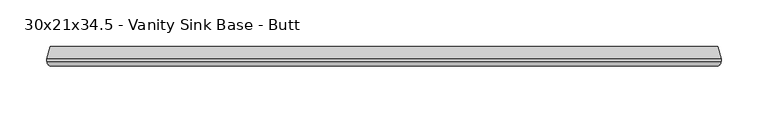
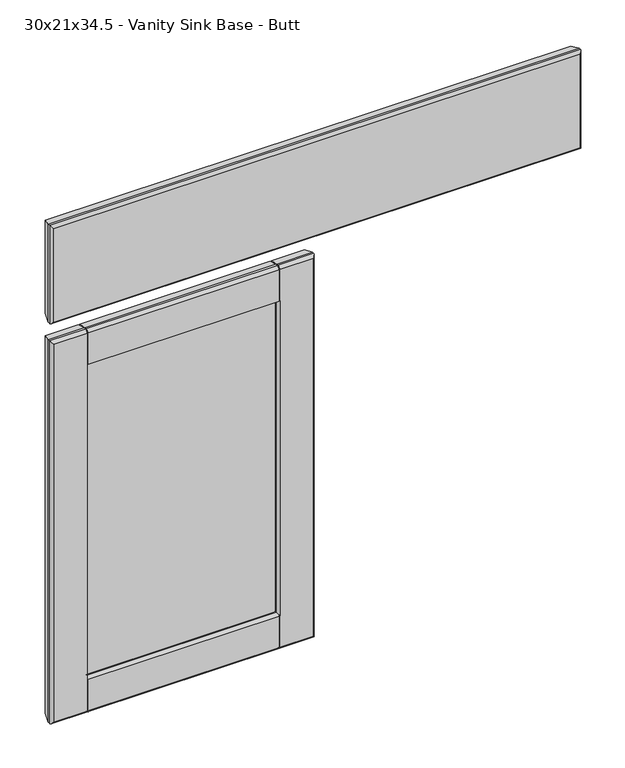
"""IFC4 building model written with IfcOpenShell, lengths in millimetres: furniture geometry, Cabinet-Base-Merillat-Double_Door-Marlin : 30x21x34.5 - Vanity Sink Base - Butt."""

from ifc_helpers import new_model, si_unit, frame, origin, place, context, project, spatial, polyline, circle_curve, ellipse_curve, outline, extrude, source, transform, mapped, element, save
from ifc_brep_helpers import plane_surface, cylinder_surface, advanced_brep


def furniture_30x21x34_5_vanity_sink_base_butt_accc5f2d(model_context):
    return source(origin(), model_context, "Body", "SolidModel", [
        advanced_brep(
        [(-336.9408026, -629.92, 847.8035075), (-336.9408026, -629.92, 714.2964925), (374.4162124, -629.92, 714.2964925), (374.4162124, -629.92, 847.8035075), (-336.5320951, -609.6, 714.7052), (-336.5320951, -609.6, 847.3948), (374.0075049, -609.6, 847.3948), (374.0075049, -609.6, 714.7052), (-340.0372951, -625.4496, 850.9), (-340.0372951, -622.681, 850.9), (-340.0372951, -622.681, 711.2), (-340.0372951, -625.4496, 711.2), (377.5127049, -622.681, 711.2), (377.5127049, -625.4496, 711.2), (377.5127049, -622.681, 850.9), (377.5127049, -625.4496, 850.9)],
        [
            (0, 1),
            (1, 2),
            (2, 3),
            (3, 0),
            (4, 5),
            (5, 6),
            (6, 7),
            (7, 4),
            (8, 9),
            (9, 10),
            (10, 11),
            (11, 8),
            (10, 12),
            (12, 13),
            (13, 11),
            (12, 14),
            (14, 15),
            (15, 13),
            (8, 15),
            (14, 9),
            (11, 1, ellipse_curve(frame((-335.2620951, -625.4496, 715.9752), z_axis=(-0.7071067811865475, 0.0, 0.7071067811865475), x_axis=(-0.7071067811865474, 0.0, -0.7071067811865476)), 6.7531526, 4.7752)),
            (0, 8, ellipse_curve(frame((-335.2620951, -625.4496, 846.1248), z_axis=(-0.7071067811865475, 0.0, -0.7071067811865475), x_axis=(0.7071067811865474, 0.0, -0.7071067811865476)), 6.7531526, 4.7752)),
            (4, 10),
            (9, 5),
            (13, 2, ellipse_curve(frame((372.7375049, -625.4496, 715.9752), z_axis=(-0.7071067811865475, 0.0, -0.7071067811865475), x_axis=(0.7071067811865476, 0.0, -0.7071067811865474)), 6.7531526, 4.7752)),
            (7, 12),
            (15, 3, ellipse_curve(frame((372.7375049, -625.4496, 846.1248), z_axis=(0.7071067811865475, 0.0, -0.7071067811865475), x_axis=(0.7071067811865474, 0.0, 0.7071067811865476)), 6.7531526, 4.7752)),
            (6, 14),
        ],
        [
            plane_surface(frame((-340.0372951, -629.92, 850.9), z_axis=(0.0, -1.0, 0.0), x_axis=(0.0, 0.0, -1.0))),
            plane_surface(frame((-340.0372951, -609.6, 850.9), z_axis=(0.0, 1.0, 0.0), x_axis=(0.0, 0.0, 1.0))),
            plane_surface(frame((-340.0372951, -629.92, 850.9), z_axis=(-1.0, 0.0, 0.0), x_axis=(0.0, 1.0, 0.0))),
            plane_surface(frame((-340.0372951, -629.92, 711.2), z_axis=(0.0, 0.0, -1.0), x_axis=(0.0, 1.0, 0.0))),
            plane_surface(frame((377.5127049, -629.92, 711.2), z_axis=(1.0, 0.0, 0.0), x_axis=(0.0, 1.0, 0.0))),
            plane_surface(frame((377.5127049, -629.92, 850.9), z_axis=(0.0, 0.0, 1.0), x_axis=(0.0, 1.0, 0.0))),
            cylinder_surface(frame((-335.2620951, -625.4496, 850.9), z_axis=(0.0, 0.0, -1.0), x_axis=(0.0, 1.0, 0.0)), 4.7752),
            plane_surface(frame((-340.0372951, -622.681, 850.9), z_axis=(-0.9659229350723619, 0.25882983502910506, 0.0), x_axis=(0.0, 0.0, -1.0))),
            cylinder_surface(frame((-340.0372951, -625.4496, 715.9752), z_axis=(1.0, 0.0, 0.0), x_axis=(0.0, 1.0, 0.0)), 4.7752),
            plane_surface(frame((-340.0372951, -622.681, 711.2), z_axis=(0.0, 0.25882983502910506, -0.9659229350723619), x_axis=(1.0, 0.0, 0.0))),
            cylinder_surface(frame((372.7375049, -625.4496, 711.2), z_axis=(0.0, 0.0, 1.0), x_axis=(0.0, 1.0, 0.0)), 4.7752),
            plane_surface(frame((377.5127049, -622.681, 711.2), z_axis=(0.9659229350723619, 0.25882983502910506, 0.0), x_axis=(0.0, 0.0, 1.0))),
            cylinder_surface(frame((377.5127049, -625.4496, 846.1248), z_axis=(-1.0, 0.0, 0.0), x_axis=(0.0, 1.0, 0.0)), 4.7752),
            plane_surface(frame((377.5127049, -622.681, 850.9), z_axis=(0.0, 0.25882983502910506, 0.9659229350723619), x_axis=(-1.0, 0.0, 0.0))),
        ],
        [
            (0, [[1, 2, 3, 4]]),
            (1, [[5, 6, 7, 8]]),
            (2, [[9, 10, 11, 12]]),
            (3, [[-11, 13, 14, 15]]),
            (4, [[-14, 16, 17, 18]]),
            (5, [[-9, 19, -17, 20]]),
            (6, [[21, -1, 22, -12]]),
            (7, [[23, -10, 24, -5]]),
            (8, [[-21, -15, 25, -2]]),
            (9, [[-23, -8, 26, -13]]),
            (10, [[-25, -18, 27, -3]]),
            (11, [[-26, -7, 28, -16]]),
            (12, [[-22, -4, -27, -19]]),
            (13, [[-24, -20, -28, -6]]),
        ],
    ),
        advanced_brep(
        [(-340.0372951, -625.4496, 685.8), (-340.0372951, -625.4496, 139.7), (-336.9408026, -629.92, 142.7964925), (-336.9408026, -629.92, 682.7035075), (-340.0372951, -622.681, 685.8), (-340.0372951, -622.681, 139.7), (-336.5320951, -609.6, 682.2948), (-336.5320951, -609.6, 143.2052), (-291.8361323, -609.6, 637.5988372), (-291.4660006, -610.39375, 637.2287055), (-289.3848416, -614.85681, 635.1475465), (-289.3848416, -614.85681, 190.3524535), (-291.4660006, -610.39375, 188.2712945), (-291.8361323, -609.6, 187.9011628), (-290.784611, -617.0969093, 636.547316), (-290.784611, -617.0969093, 188.952684), (-305.1122951, -617.347, 650.875), (-305.1122951, -617.347, 174.625), (-305.1122951, -622.173, 650.875), (-305.1122951, -622.173, 174.625), (-290.784611, -622.4230907, 636.547316), (-290.784611, -622.4230907, 188.952684), (-289.3848416, -624.66319, 635.1475465), (-289.3848416, -624.66319, 190.3524535), (-291.4660006, -629.12625, 637.2287055), (-291.8332649, -629.9138508, 637.5959698), (-291.8361323, -629.92, 187.9011628), (-291.4660006, -629.12625, 188.2712945), (14.0537124, -629.92, 142.7964925), (-31.0140137, -629.92, 142.7964925), (-31.0140137, -625.4496, 139.7), (17.1502049, -625.4496, 139.7), (-291.8332649, -625.4496, 139.7), (-291.8332649, -629.92, 142.7964925), (-290.2457649, -625.4496, 139.7), (-32.6015137, -625.4496, 139.7), (-32.6015137, -629.92, 142.7964925), (-290.2457649, -629.92, 142.7964925), (-31.0140137, -622.681, 139.7), (17.1502049, -622.681, 139.7), (-291.8332649, -622.681, 139.7), (-290.2457649, -622.681, 139.7), (-32.6015137, -622.681, 139.7), (-31.0140137, -609.6, 143.2052), (13.6450049, -609.6, 143.2052), (-290.2457649, -609.6, 143.2052), (-32.6015137, -609.6, 143.2052), (-291.8332649, -609.6, 143.2052), (-33.5022486, -614.85681, 190.3524535), (-31.4210895, -610.39375, 188.2712945), (-32.6015137, -610.39375, 188.2712945), (-32.6015137, -609.6, 187.9011628), (-290.2457649, -609.6, 187.9011628), (-290.2457649, -610.39375, 188.2712945), (-32.1024791, -617.0969093, 188.952684), (-17.7747951, -617.347, 174.625), (-17.7747951, -622.173, 174.625), (-32.1024791, -622.4230907, 188.952684), (-33.5022486, -624.66319, 190.3524535), (-290.2457649, -629.12625, 188.2712945), (-290.2457649, -629.92, 187.9011628), (-32.6015137, -629.92, 187.9011628), (-32.6015137, -629.12625, 188.2712945), (-31.4210895, -629.12625, 188.2712945), (17.1502049, -625.4496, 685.8), (14.0537124, -629.92, 682.7035075), (17.1502049, -622.681, 685.8), (13.6450049, -609.6, 682.2948), (-31.0509578, -609.6, 187.9011628), (-33.5022486, -614.85681, 635.1475465), (-31.4210895, -610.39375, 637.2287055), (-31.0509578, -609.6, 637.5988372), (-32.1024791, -617.0969093, 636.547316), (-17.7747951, -617.347, 650.875), (-17.7747951, -622.173, 650.875), (-32.1024791, -622.4230907, 636.547316), (-33.5022486, -624.66319, 635.1475465), (-31.0509578, -629.92, 187.9011628), (-31.0509578, -629.92, 637.5988372), (-31.4210895, -629.12625, 637.2287055), (-291.8332649, -629.92, 682.7035075), (-291.8332649, -625.4496, 685.8), (-31.0140137, -625.4496, 685.8), (-31.0140137, -629.92, 682.7035075), (-32.6015137, -625.4496, 685.8), (-290.2457649, -625.4496, 685.8), (-290.2457649, -629.92, 682.7035075), (-32.6015137, -629.92, 682.7035075), (-291.8332649, -622.681, 685.8), (-31.0140137, -622.681, 685.8), (-32.6015137, -622.681, 685.8), (-290.2457649, -622.681, 685.8), (-291.8332649, -609.6, 682.2948), (-31.0140137, -609.6, 682.2948), (-32.6015137, -609.6, 682.2948), (-290.2457649, -609.6, 682.2948), (-32.6015137, -609.6, 637.5988372), (-290.2457649, -609.6, 637.5988372), (-290.2457649, -610.39375, 637.2287055), (-32.6015137, -610.39375, 637.2287055), (-32.6015137, -629.12625, 637.2287055), (-32.6015137, -629.92, 637.5988372), (-290.2457649, -629.92, 637.5988372), (-290.2457649, -629.12625, 637.2287055), (-32.6015137, -629.12625, 682.5526052), (-32.6015137, -625.4496, 685.00625), (-32.6015137, -622.7855037, 685.00625), (-32.6015137, -610.39375, 681.6857412), (-31.0140137, -610.39375, 637.2287055), (-31.0140137, -610.39375, 681.6857412), (-31.0140137, -622.7855037, 685.00625), (-31.0140137, -625.4496, 685.00625), (-31.0140137, -629.12625, 682.5526052), (-31.0140137, -629.12625, 637.2287055), (-291.8332649, -629.12625, 637.2287055), (-291.8332649, -629.12625, 682.5526052), (-291.8332649, -625.4496, 685.00625), (-291.8332649, -622.7855037, 685.00625), (-291.8332649, -610.39375, 681.6857412), (-291.8332649, -610.39375, 637.2287055), (-290.2457649, -610.39375, 681.6857412), (-290.2457649, -622.7855037, 685.00625), (-290.2457649, -625.4496, 685.00625), (-290.2457649, -629.12625, 682.5526052), (-291.8332649, -610.39375, 188.2712945), (-291.8332649, -610.39375, 143.8142588), (-291.8332649, -622.7855037, 140.49375), (-291.8332649, -625.4496, 140.49375), (-291.8332649, -629.12625, 142.9473948), (-291.8332649, -629.12625, 188.2712945), (-290.2457649, -629.12625, 142.9473948), (-290.2457649, -625.4496, 140.49375), (-290.2457649, -622.7855037, 140.49375), (-290.2457649, -610.39375, 143.8142588), (-32.6015137, -610.39375, 143.8142588), (-32.6015137, -622.7855037, 140.49375), (-32.6015137, -625.4496, 140.49375), (-32.6015137, -629.12625, 142.9473948), (-31.0140137, -629.12625, 188.2712945), (-31.0140137, -629.12625, 142.9473948), (-31.0140137, -625.4496, 140.49375), (-31.0140137, -622.7855037, 140.49375), (-31.0140137, -610.39375, 143.8142588), (-31.0140137, -610.39375, 188.2712945)],
        [
            (0, 1),
            (1, 2, ellipse_curve(frame((-335.2620951, -625.4496, 144.4752), z_axis=(-0.7071067811865475, 0.0, 0.7071067811865475), x_axis=(0.7071067811865474, 0.0, 0.7071067811865476)), 6.7531526, 4.7752)),
            (2, 3),
            (3, 0, ellipse_curve(frame((-335.2620951, -625.4496, 681.0248), z_axis=(-0.7071067811865475, 0.0, -0.7071067811865475), x_axis=(-0.7071067811865474, 0.0, 0.7071067811865476)), 6.7531526, 4.7752)),
            (0, 4),
            (4, 5),
            (5, 1),
            (4, 6),
            (6, 7),
            (7, 5),
            (8, 9),
            (9, 10),
            (10, 11),
            (11, 12),
            (12, 13),
            (13, 8),
            (10, 14, ellipse_curve(frame((-290.8120951, -615.5223492, 636.5748), z_axis=(-0.7071067811865475, 0.0, -0.7071067811865475), x_axis=(-0.7071067811865474, 0.0, 0.7071067811865476)), 2.2271035, 1.5748)),
            (14, 15),
            (15, 11, ellipse_curve(frame((-290.8120951, -615.5223492, 188.9252), z_axis=(-0.7071067811865475, 0.0, 0.7071067811865475), x_axis=(0.7071067811865474, 0.0, 0.7071067811865476)), 2.2271035, 1.5748)),
            (14, 16),
            (16, 17),
            (17, 15),
            (16, 18),
            (18, 19),
            (19, 17),
            (18, 20),
            (20, 21),
            (21, 19),
            (20, 22, ellipse_curve(frame((-290.8120951, -623.9976508, 636.5748), z_axis=(-0.7071067811865475, 0.0, -0.7071067811865475), x_axis=(-0.7071067811865474, 0.0, 0.7071067811865476)), 2.2271035, 1.5748)),
            (22, 23),
            (23, 21, ellipse_curve(frame((-290.8120951, -623.9976508, 188.9252), z_axis=(-0.7071067811865475, 0.0, 0.7071067811865475), x_axis=(0.7071067811865474, 0.0, 0.7071067811865476)), 2.2271035, 1.5748)),
            (22, 24),
            (24, 25),
            (25, 26),
            (26, 27),
            (27, 23),
            (28, 29),
            (29, 30, circle_curve(frame((-31.0140137, -625.4496, 144.4752), z_axis=(1.0, 0.0, 0.0), x_axis=(0.0, 1.0, 0.0)), 4.7752)),
            (30, 31),
            (31, 28, ellipse_curve(frame((12.3750049, -625.4496, 144.4752), z_axis=(-0.7071067811865475, 0.0, -0.7071067811865475), x_axis=(-0.7071067811865476, 0.0, 0.7071067811865474)), 6.7531526, 4.7752)),
            (1, 32),
            (32, 33, circle_curve(frame((-291.8332649, -625.4496, 144.4752), z_axis=(-1.0, 0.0, 0.0), x_axis=(0.0, 1.0, 0.0)), 4.7752)),
            (33, 2),
            (34, 35),
            (35, 36, circle_curve(frame((-32.6015137, -625.4496, 144.4752), z_axis=(-1.0, 0.0, 0.0), x_axis=(0.0, 1.0, 0.0)), 4.7752)),
            (36, 37),
            (37, 34, circle_curve(frame((-290.2457649, -625.4496, 144.4752), z_axis=(1.0, 0.0, 0.0), x_axis=(0.0, 1.0, 0.0)), 4.7752)),
            (30, 38),
            (38, 39),
            (39, 31),
            (5, 40),
            (40, 32),
            (41, 42),
            (42, 35),
            (34, 41),
            (38, 43),
            (43, 44),
            (44, 39),
            (45, 46),
            (46, 42),
            (41, 45),
            (7, 47),
            (47, 40),
            (48, 49),
            (49, 50),
            (50, 51),
            (51, 52),
            (52, 53),
            (53, 12),
            (11, 48),
            (15, 54),
            (54, 48, ellipse_curve(frame((-32.0749951, -615.5223492, 188.9252), z_axis=(-0.7071067811865475, 0.0, -0.7071067811865475), x_axis=(-0.7071067811865476, 0.0, 0.7071067811865474)), 2.2271035, 1.5748)),
            (17, 55),
            (55, 54),
            (19, 56),
            (56, 55),
            (21, 57),
            (57, 56),
            (23, 58),
            (58, 57, ellipse_curve(frame((-32.0749951, -623.9976508, 188.9252), z_axis=(-0.7071067811865475, 0.0, -0.7071067811865475), x_axis=(-0.7071067811865476, 0.0, 0.7071067811865474)), 2.2271035, 1.5748)),
            (27, 59),
            (59, 60),
            (60, 61),
            (61, 62),
            (62, 63),
            (63, 58),
            (31, 64),
            (64, 65, ellipse_curve(frame((12.3750049, -625.4496, 681.0248), z_axis=(0.7071067811865475, 0.0, -0.7071067811865475), x_axis=(-0.7071067811865474, 0.0, -0.7071067811865476)), 6.7531526, 4.7752)),
            (65, 28),
            (39, 66),
            (66, 64),
            (44, 67),
            (67, 66),
            (68, 49),
            (48, 69),
            (69, 70),
            (70, 71),
            (71, 68),
            (54, 72),
            (72, 69, ellipse_curve(frame((-32.0749951, -615.5223492, 636.5748), z_axis=(0.7071067811865475, 0.0, -0.7071067811865475), x_axis=(-0.7071067811865474, 0.0, -0.7071067811865476)), 2.2271035, 1.5748)),
            (55, 73),
            (73, 72),
            (56, 74),
            (74, 73),
            (57, 75),
            (75, 74),
            (58, 76),
            (76, 75, ellipse_curve(frame((-32.0749951, -623.9976508, 636.5748), z_axis=(0.7071067811865475, 0.0, -0.7071067811865475), x_axis=(-0.7071067811865474, 0.0, -0.7071067811865476)), 2.2271035, 1.5748)),
            (63, 77),
            (77, 78),
            (78, 79),
            (79, 76),
            (3, 80),
            (80, 81, circle_curve(frame((-291.8332649, -625.4496, 681.0248), z_axis=(-1.0, 0.0, 0.0), x_axis=(0.0, 1.0, 0.0)), 4.7752)),
            (81, 0),
            (64, 82),
            (82, 83, circle_curve(frame((-31.0140137, -625.4496, 681.0248), z_axis=(1.0, 0.0, 0.0), x_axis=(0.0, 1.0, 0.0)), 4.7752)),
            (83, 65),
            (84, 85),
            (85, 86, circle_curve(frame((-290.2457649, -625.4496, 681.0248), z_axis=(1.0, 0.0, 0.0), x_axis=(0.0, 1.0, 0.0)), 4.7752)),
            (86, 87),
            (87, 84, circle_curve(frame((-32.6015137, -625.4496, 681.0248), z_axis=(-1.0, 0.0, 0.0), x_axis=(0.0, 1.0, 0.0)), 4.7752)),
            (81, 88),
            (88, 4),
            (66, 89),
            (89, 82),
            (90, 91),
            (91, 85),
            (84, 90),
            (88, 92),
            (92, 6),
            (67, 93),
            (93, 89),
            (94, 95),
            (95, 91),
            (90, 94),
            (51, 46),
            (45, 52),
            (43, 68),
            (71, 93),
            (92, 8),
            (13, 47),
            (96, 97),
            (97, 95),
            (94, 96),
            (9, 98),
            (98, 97),
            (96, 99),
            (99, 70),
            (69, 10),
            (72, 14),
            (73, 16),
            (74, 18),
            (75, 20),
            (76, 22),
            (79, 100),
            (100, 101),
            (101, 102),
            (102, 103),
            (103, 24),
            (33, 26),
            (25, 80),
            (36, 61),
            (60, 37),
            (83, 78),
            (77, 29),
            (86, 102),
            (101, 87),
            (100, 104),
            (104, 105, circle_curve(frame((-32.6015137, -625.4496, 681.0248), z_axis=(-1.0, 0.0, 0.0), x_axis=(0.0, 0.0, 1.0)), 3.98145)),
            (105, 106),
            (106, 107),
            (107, 99),
            (71, 108),
            (108, 109),
            (109, 110),
            (110, 111),
            (111, 112, circle_curve(frame((-31.0140137, -625.4496, 681.0248), z_axis=(1.0, 0.0, 0.0), x_axis=(0.0, 0.0, 1.0)), 3.98145)),
            (112, 113),
            (113, 78),
            (113, 79),
            (112, 104),
            (111, 105),
            (110, 106),
            (109, 107),
            (108, 70),
            (25, 114),
            (114, 115),
            (115, 116, circle_curve(frame((-291.8332649, -625.4496, 681.0248), z_axis=(-1.0, 0.0, 0.0), x_axis=(0.0, 0.0, 1.0)), 3.98145)),
            (116, 117),
            (117, 118),
            (118, 119),
            (119, 8),
            (98, 120),
            (120, 121),
            (121, 122),
            (122, 123, circle_curve(frame((-290.2457649, -625.4496, 681.0248), z_axis=(1.0, 0.0, 0.0), x_axis=(0.0, 0.0, 1.0)), 3.98145)),
            (123, 103),
            (24, 114),
            (123, 115),
            (122, 116),
            (121, 117),
            (120, 118),
            (9, 119),
            (13, 124),
            (124, 125),
            (125, 126),
            (126, 127),
            (127, 128, circle_curve(frame((-291.8332649, -625.4496, 144.4752), z_axis=(-1.0, 0.0, 0.0), x_axis=(0.0, 0.0, 1.0)), 3.98145)),
            (128, 129),
            (129, 26),
            (59, 130),
            (130, 131, circle_curve(frame((-290.2457649, -625.4496, 144.4752), z_axis=(1.0, 0.0, 0.0), x_axis=(0.0, 0.0, 1.0)), 3.98145)),
            (131, 132),
            (132, 133),
            (133, 53),
            (12, 124),
            (133, 125),
            (132, 126),
            (131, 127),
            (130, 128),
            (27, 129),
            (50, 134),
            (134, 135),
            (135, 136),
            (136, 137, circle_curve(frame((-32.6015137, -625.4496, 144.4752), z_axis=(-1.0, 0.0, 0.0), x_axis=(0.0, 0.0, 1.0)), 3.98145)),
            (137, 62),
            (138, 139),
            (139, 140, circle_curve(frame((-31.0140137, -625.4496, 144.4752), z_axis=(1.0, 0.0, 0.0), x_axis=(0.0, 0.0, 1.0)), 3.98145)),
            (140, 141),
            (141, 142),
            (142, 143),
            (143, 68),
            (77, 138),
            (63, 138),
            (143, 49),
            (142, 134),
            (141, 135),
            (140, 136),
            (139, 137),
        ],
        [
            cylinder_surface(frame((-335.2620951, -625.4496, 685.8), z_axis=(0.0, 0.0, 1.0), x_axis=(0.0, 1.0, 0.0)), 4.7752),
            plane_surface(frame((-340.0372951, -625.4496, 685.8), z_axis=(-1.0, 0.0, 0.0), x_axis=(0.0, 0.0, -1.0))),
            plane_surface(frame((-340.0372951, -622.681, 685.8), z_axis=(-0.9659229350723619, 0.25882983502910506, 0.0), x_axis=(0.0, 0.0, -1.0))),
            plane_surface(frame((-291.8361323, -609.6, 637.5988372), z_axis=(0.9063077870366099, 0.4226182617407856, 0.0), x_axis=(0.0, 0.0, -1.0))),
            cylinder_surface(frame((-290.8120951, -615.5223492, 685.8), z_axis=(0.0, 0.0, 1.0000000000000002), x_axis=(0.01745240643729364, -0.9998476951563912, 0.0)), 1.5748),
            plane_surface(frame((-290.784611, -617.0969093, 636.547316), z_axis=(0.017452406437322144, -0.9998476951563906, 0.0), x_axis=(0.0, 0.0, -1.0))),
            plane_surface(frame((-305.1122951, -617.347, 650.875), z_axis=(1.0, 0.0, 0.0), x_axis=(0.0, 0.0, -1.0))),
            plane_surface(frame((-305.1122951, -622.173, 650.875), z_axis=(0.01745240643727848, 0.9998476951563914, 0.0), x_axis=(0.0, 0.0, -1.0))),
            cylinder_surface(frame((-290.8120951, -623.9976508, 685.8), z_axis=(0.0, 0.0, 1.0000000000000002), x_axis=(0.9063077870367326, -0.42261826174052236, 0.0)), 1.5748),
            plane_surface(frame((-289.3848416, -624.66319, 635.1475465), z_axis=(0.9063077870366333, -0.4226182617407352, 0.0), x_axis=(0.0, 0.0, -1.0))),
            cylinder_surface(frame((-340.0372951, -625.4496, 144.4752), z_axis=(-1.0, 0.0, 0.0), x_axis=(0.0, 1.0, 0.0)), 4.7752),
            plane_surface(frame((-340.0372951, -625.4496, 139.7), z_axis=(0.0, 0.0, -1.0), x_axis=(1.0, 0.0, 0.0))),
            plane_surface(frame((-340.0372951, -622.681, 139.7), z_axis=(0.0, 0.25882983502910506, -0.9659229350723619), x_axis=(1.0, 0.0, 0.0))),
            plane_surface(frame((-291.8361323, -609.6, 187.9011628), z_axis=(0.0, 0.4226182617407856, 0.9063077870366099), x_axis=(1.0, 0.0, 0.0))),
            cylinder_surface(frame((-340.0372951, -615.5223492, 188.9252), z_axis=(-1.0000000000000002, 0.0, 0.0), x_axis=(0.0, -0.9998476951563912, 0.01745240643729364)), 1.5748),
            plane_surface(frame((-290.784611, -617.0969093, 188.952684), z_axis=(0.0, -0.9998476951563906, 0.017452406437322144), x_axis=(1.0, 0.0, 0.0))),
            plane_surface(frame((-305.1122951, -617.347, 174.625), z_axis=(0.0, 0.0, 1.0), x_axis=(1.0, 0.0, 0.0))),
            plane_surface(frame((-305.1122951, -622.173, 174.625), z_axis=(0.0, 0.9998476951563914, 0.01745240643727848), x_axis=(1.0, 0.0, 0.0))),
            cylinder_surface(frame((-340.0372951, -623.9976508, 188.9252), z_axis=(-1.0000000000000002, 0.0, 0.0), x_axis=(0.0, -0.42261826174052236, 0.9063077870367326)), 1.5748),
            plane_surface(frame((-289.3848416, -624.66319, 190.3524535), z_axis=(0.0, -0.4226182617407352, 0.9063077870366333), x_axis=(1.0, 0.0, 0.0))),
            cylinder_surface(frame((12.3750049, -625.4496, 139.7), z_axis=(0.0, 0.0, -1.0), x_axis=(0.0, 1.0, 0.0)), 4.7752),
            plane_surface(frame((17.1502049, -625.4496, 139.7), z_axis=(1.0, 0.0, 0.0), x_axis=(0.0, 0.0, 1.0))),
            plane_surface(frame((17.1502049, -622.681, 139.7), z_axis=(0.9659229350723619, 0.25882983502910506, 0.0), x_axis=(0.0, 0.0, 1.0))),
            plane_surface(frame((-31.0509578, -609.6, 187.9011628), z_axis=(-0.9063077870366099, 0.4226182617407856, 0.0), x_axis=(0.0, 0.0, 1.0))),
            cylinder_surface(frame((-32.0749951, -615.5223492, 139.7), z_axis=(0.0, 0.0, -1.0000000000000002), x_axis=(-0.01745240643729364, -0.9998476951563912, 0.0)), 1.5748),
            plane_surface(frame((-32.1024791, -617.0969093, 188.952684), z_axis=(-0.017452406437322144, -0.9998476951563906, 0.0), x_axis=(0.0, 0.0, 1.0))),
            plane_surface(frame((-17.7747951, -617.347, 174.625), z_axis=(-1.0, 0.0, 0.0), x_axis=(0.0, 0.0, 1.0))),
            plane_surface(frame((-17.7747951, -622.173, 174.625), z_axis=(-0.01745240643727848, 0.9998476951563914, 0.0), x_axis=(0.0, 0.0, 1.0))),
            cylinder_surface(frame((-32.0749951, -623.9976508, 139.7), z_axis=(0.0, 0.0, -1.0000000000000002), x_axis=(-0.9063077870367326, -0.42261826174052236, 0.0)), 1.5748),
            plane_surface(frame((-33.5022486, -624.66319, 190.3524535), z_axis=(-0.9063077870366333, -0.4226182617407352, 0.0), x_axis=(0.0, 0.0, 1.0))),
            cylinder_surface(frame((17.1502049, -625.4496, 681.0248), z_axis=(1.0, 0.0, 0.0), x_axis=(0.0, 1.0, 0.0)), 4.7752),
            plane_surface(frame((17.1502049, -625.4496, 685.8), z_axis=(0.0, 0.0, 1.0), x_axis=(-1.0, 0.0, 0.0))),
            plane_surface(frame((17.1502049, -622.681, 685.8), z_axis=(0.0, 0.25882983502910506, 0.9659229350723619), x_axis=(-1.0, 0.0, 0.0))),
            plane_surface(frame((13.6450049, -609.6, 682.2948), z_axis=(0.0, 1.0, 0.0), x_axis=(-1.0, 0.0, 0.0))),
            plane_surface(frame((-31.0509578, -609.6, 637.5988372), z_axis=(0.0, 0.4226182617407856, -0.9063077870366099), x_axis=(-1.0, 0.0, 0.0))),
            cylinder_surface(frame((17.1502049, -615.5223492, 636.5748), z_axis=(1.0000000000000002, 0.0, 0.0), x_axis=(0.0, -0.9998476951563912, -0.01745240643729364)), 1.5748),
            plane_surface(frame((-32.1024791, -617.0969093, 636.547316), z_axis=(0.0, -0.9998476951563906, -0.017452406437322144), x_axis=(-1.0, 0.0, 0.0))),
            plane_surface(frame((-17.7747951, -617.347, 650.875), z_axis=(0.0, 0.0, -1.0), x_axis=(-1.0, 0.0, 0.0))),
            plane_surface(frame((-17.7747951, -622.173, 650.875), z_axis=(0.0, 0.9998476951563914, -0.01745240643727848), x_axis=(-1.0, 0.0, 0.0))),
            cylinder_surface(frame((17.1502049, -623.9976508, 636.5748), z_axis=(1.0000000000000002, 0.0, 0.0), x_axis=(0.0, -0.42261826174052236, -0.9063077870367326)), 1.5748),
            plane_surface(frame((-33.5022486, -624.66319, 635.1475465), z_axis=(0.0, -0.4226182617407352, -0.9063077870366333), x_axis=(-1.0, 0.0, 0.0))),
            plane_surface(frame((-31.0509578, -629.92, 637.5988372), z_axis=(0.0, -1.0, 0.0), x_axis=(-1.0, 0.0, 0.0))),
            plane_surface(frame((-32.6015137, -629.92, 637.5988372), z_axis=(1.0, 0.0, 0.0), x_axis=(0.0, 0.906307787036771, -0.4226182617404399))),
            plane_surface(frame((-31.0140137, -629.92, 637.5988372), z_axis=(-1.0, 0.0, 0.0), x_axis=(0.0, -0.906307787036771, 0.4226182617404399))),
            plane_surface(frame((-32.6015137, -629.92, 637.5988372), z_axis=(0.0, 0.4226182617404399, 0.906307787036771), x_axis=(1.0, 0.0, 0.0))),
            plane_surface(frame((-32.6015137, -629.12625, 637.2287055), z_axis=(0.0, -1.0, 0.0), x_axis=(1.0, 0.0, 0.0))),
            cylinder_surface(frame((-31.0140137, -625.4496, 681.0248), z_axis=(1.0, 0.0, 0.0), x_axis=(0.0, 0.0, 1.0)), 3.98145),
            plane_surface(frame((-32.6015137, -625.4496, 685.00625), z_axis=(0.0, 0.0, 1.0), x_axis=(1.0, 0.0, 0.0))),
            plane_surface(frame((-32.6015137, -622.7855037, 685.00625), z_axis=(0.0, 0.25882983502913415, 0.9659229350723542), x_axis=(1.0, 0.0, 0.0))),
            plane_surface(frame((-32.6015137, -610.39375, 681.6857412), z_axis=(0.0, 1.0, 0.0), x_axis=(1.0, 0.0, 0.0))),
            plane_surface(frame((-32.6015137, -610.39375, 637.2287055), z_axis=(0.0, -0.4226182617405111, 0.9063077870367379), x_axis=(1.0, 0.0, 0.0))),
            plane_surface(frame((-291.8332649, -629.92, 637.5988372), z_axis=(1.0, 0.0, 0.0), x_axis=(0.0, 0.9063077870367783, -0.42261826174042444))),
            plane_surface(frame((-290.2457649, -629.92, 637.5988372), z_axis=(-1.0, 0.0, 0.0), x_axis=(0.0, -0.9063077870367783, 0.42261826174042444))),
            plane_surface(frame((-291.8332649, -629.92, 637.5988372), z_axis=(0.0, 0.42261826174042444, 0.9063077870367783), x_axis=(1.0, 0.0, 0.0))),
            plane_surface(frame((-291.8332649, -629.12625, 637.2287055), z_axis=(0.0, -1.0, 0.0), x_axis=(1.0, 0.0, 0.0))),
            cylinder_surface(frame((-290.2457649, -625.4496, 681.0248), z_axis=(1.0, 0.0, 0.0), x_axis=(0.0, 0.0, 1.0)), 3.98145),
            plane_surface(frame((-291.8332649, -625.4496, 685.00625), z_axis=(0.0, 0.0, 1.0), x_axis=(1.0, 0.0, 0.0))),
            plane_surface(frame((-291.8332649, -622.7855037, 685.00625), z_axis=(0.0, 0.25882983502911566, 0.965922935072359), x_axis=(1.0, 0.0, 0.0))),
            plane_surface(frame((-291.8332649, -610.39375, 681.6857412), z_axis=(0.0, 1.0, 0.0), x_axis=(1.0, 0.0, 0.0))),
            plane_surface(frame((-291.8332649, -610.39375, 637.2287055), z_axis=(0.0, -0.42261826174056427, 0.9063077870367131), x_axis=(1.0, 0.0, 0.0))),
            plane_surface(frame((-291.8332649, -625.4496, 149.2504), z_axis=(1.0, 0.0, 0.0), x_axis=(0.0, -1.0, 0.0))),
            plane_surface(frame((-290.2457649, -625.4496, 149.2504), z_axis=(-1.0, 0.0, 0.0), x_axis=(0.0, 1.0, 0.0))),
            plane_surface(frame((-291.8332649, -609.6, 187.9011628), z_axis=(0.0, -0.42261826173999295, -0.9063077870369795), x_axis=(1.0, 0.0, 0.0))),
            plane_surface(frame((-291.8332649, -610.39375, 188.2712945), z_axis=(0.0, 1.0, 0.0), x_axis=(1.0, 0.0, 0.0))),
            plane_surface(frame((-291.8332649, -610.39375, 143.8142588), z_axis=(0.0, 0.2588298350290845, -0.9659229350723675), x_axis=(1.0, 0.0, 0.0))),
            plane_surface(frame((-291.8332649, -622.7855037, 140.49375), z_axis=(0.0, 0.0, -1.0), x_axis=(1.0, 0.0, 0.0))),
            cylinder_surface(frame((-290.2457649, -625.4496, 144.4752), z_axis=(1.0, 0.0, 0.0), x_axis=(0.0, 0.0, 1.0)), 3.98145),
            plane_surface(frame((-291.8332649, -629.12625, 142.9473948), z_axis=(0.0, -1.0, 0.0), x_axis=(1.0, 0.0, 0.0))),
            plane_surface(frame((-291.8332649, -629.12625, 188.2712945), z_axis=(0.0, 0.4226182617407698, -0.9063077870366172), x_axis=(1.0, 0.0, 0.0))),
            plane_surface(frame((-32.6015137, -629.12625, 188.2712945), z_axis=(1.0, 0.0, 0.0), x_axis=(0.0, -0.906307787036583, -0.42261826174084305))),
            plane_surface(frame((-31.0140137, -629.12625, 188.2712945), z_axis=(-1.0, 0.0, 0.0), x_axis=(0.0, 0.906307787036583, 0.42261826174084305))),
            plane_surface(frame((-32.6015137, -629.12625, 188.2712945), z_axis=(0.0, 0.42261826174084305, -0.906307787036583), x_axis=(1.0, 0.0, 0.0))),
            plane_surface(frame((-32.6015137, -609.6, 187.9011628), z_axis=(0.0, -0.42261826174073325, -0.9063077870366342), x_axis=(1.0, 0.0, 0.0))),
            plane_surface(frame((-32.6015137, -610.39375, 188.2712945), z_axis=(0.0, 1.0, 0.0), x_axis=(1.0, 0.0, 0.0))),
            plane_surface(frame((-32.6015137, -610.39375, 143.8142588), z_axis=(0.0, 0.2588298350290967, -0.9659229350723642), x_axis=(1.0, 0.0, 0.0))),
            plane_surface(frame((-32.6015137, -622.7855037, 140.49375), z_axis=(0.0, 0.0, -1.0), x_axis=(1.0, 0.0, 0.0))),
            cylinder_surface(frame((-31.0140137, -625.4496, 144.4752), z_axis=(1.0, 0.0, 0.0), x_axis=(0.0, 0.0, 1.0)), 3.98145),
            plane_surface(frame((-32.6015137, -629.12625, 142.9473948), z_axis=(0.0, -1.0, 0.0), x_axis=(1.0, 0.0, 0.0))),
        ],
        [
            (0, [[1, 2, 3, 4]]),
            (1, [[5, 6, 7, -1]]),
            (2, [[8, 9, 10, -6]]),
            (3, [[11, 12, 13, 14, 15, 16]]),
            (4, [[17, 18, 19, -13]]),
            (5, [[20, 21, 22, -18]]),
            (6, [[23, 24, 25, -21]]),
            (7, [[26, 27, 28, -24]]),
            (8, [[29, 30, 31, -27]]),
            (9, [[32, 33, 34, 35, 36, -30]]),
            (10, [[37, 38, 39, 40]]),
            (10, [[41, 42, 43, -2]]),
            (10, [[44, 45, 46, 47]]),
            (11, [[-39, 48, 49, 50]]),
            (11, [[51, 52, -41, -7]]),
            (11, [[53, 54, -44, 55]]),
            (12, [[-49, 56, 57, 58]]),
            (12, [[59, 60, -53, 61]]),
            (12, [[62, 63, -51, -10]]),
            (13, [[64, 65, 66, 67, 68, 69, -14, 70]]),
            (14, [[71, 72, -70, -19]]),
            (15, [[73, 74, -71, -22]]),
            (16, [[75, 76, -73, -25]]),
            (17, [[77, 78, -75, -28]]),
            (18, [[79, 80, -77, -31]]),
            (19, [[-36, 81, 82, 83, 84, 85, 86, -79]]),
            (20, [[87, 88, 89, -40]]),
            (21, [[90, 91, -87, -50]]),
            (22, [[92, 93, -90, -58]]),
            (23, [[94, -64, 95, 96, 97, 98]]),
            (24, [[99, 100, -95, -72]]),
            (25, [[101, 102, -99, -74]]),
            (26, [[103, 104, -101, -76]]),
            (27, [[105, 106, -103, -78]]),
            (28, [[107, 108, -105, -80]]),
            (29, [[-86, 109, 110, 111, 112, -107]]),
            (30, [[113, 114, 115, -4]]),
            (30, [[116, 117, 118, -88]]),
            (30, [[119, 120, 121, 122]]),
            (31, [[-115, 123, 124, -5]]),
            (31, [[125, 126, -116, -91]]),
            (31, [[127, 128, -119, 129]]),
            (32, [[-124, 130, 131, -8]]),
            (32, [[132, 133, -125, -93]]),
            (32, [[134, 135, -127, 136]]),
            (33, [[-67, 137, -59, 138]]),
            (33, [[-57, 139, -98, 140, -132, -92]]),
            (33, [[-131, 141, -16, 142, -62, -9]]),
            (33, [[143, 144, -134, 145]]),
            (34, [[-12, 146, 147, -143, 148, 149, -96, 150]]),
            (35, [[-150, -100, 151, -17]]),
            (36, [[-151, -102, 152, -20]]),
            (37, [[-152, -104, 153, -23]]),
            (38, [[-153, -106, 154, -26]]),
            (39, [[-154, -108, 155, -29]]),
            (40, [[-112, 156, 157, 158, 159, 160, -32, -155]]),
            (41, [[-43, 161, -34, 162, -113, -3]]),
            (41, [[-46, 163, -83, 164]]),
            (41, [[-118, 165, -110, 166, -37, -89]]),
            (41, [[-121, 167, -158, 168]]),
            (42, [[-148, -145, -136, -129, -122, -168, -157, 169, 170, 171, 172, 173]]),
            (43, [[-165, -117, -126, -133, -140, 174, 175, 176, 177, 178, 179, 180]]),
            (44, [[181, -111, -180]]),
            (45, [[-156, -181, -179, 182, -169]]),
            (46, [[-182, -178, 183, -170]]),
            (47, [[-183, -177, 184, -171]]),
            (48, [[-184, -176, 185, -172]]),
            (49, [[-185, -175, 186, -149, -173]]),
            (50, [[-97, -186, -174]]),
            (51, [[-141, -130, -123, -114, -162, 187, 188, 189, 190, 191, 192, 193]]),
            (52, [[-159, -167, -120, -128, -135, -144, -147, 194, 195, 196, 197, 198]]),
            (53, [[-33, 199, -187]]),
            (54, [[-199, -160, -198, 200, -188]]),
            (55, [[-200, -197, 201, -189]]),
            (56, [[-201, -196, 202, -190]]),
            (57, [[-202, -195, 203, -191]]),
            (58, [[-203, -194, -146, 204, -192]]),
            (59, [[-204, -11, -193]]),
            (60, [[-161, -42, -52, -63, -142, 205, 206, 207, 208, 209, 210, 211]]),
            (61, [[-68, -138, -61, -55, -47, -164, -82, 212, 213, 214, 215, 216]]),
            (62, [[-15, 217, -205]]),
            (63, [[-217, -69, -216, 218, -206]]),
            (64, [[-218, -215, 219, -207]]),
            (65, [[-219, -214, 220, -208]]),
            (66, [[-220, -213, 221, -209]]),
            (67, [[-221, -212, -81, 222, -210]]),
            (68, [[-222, -35, -211]]),
            (69, [[-84, -163, -45, -54, -60, -137, -66, 223, 224, 225, 226, 227]]),
            (70, [[228, 229, 230, 231, 232, 233, -139, -56, -48, -38, -166, 234]]),
            (71, [[-109, 235, -234]]),
            (72, [[236, -94, -233]]),
            (73, [[-65, -236, -232, 237, -223]]),
            (74, [[-237, -231, 238, -224]]),
            (75, [[-238, -230, 239, -225]]),
            (76, [[-239, -229, 240, -226]]),
            (77, [[-240, -228, -235, -85, -227]]),
        ],
    ),
        extrude(outline(polyline([(-17.7747951, -622.173), (-305.1122951, -622.173), (-305.1122951, -617.347), (-17.7747951, -617.347), (-17.7747951, -622.173)])), frame((0.0, 0.0, 174.625), z_axis=(0.0, 0.0, 1.0), x_axis=(1.0, 0.0, 0.0)), (0.0, 0.0, 1.0), 476.25),
    ])


if __name__ == "__main__":
    model = new_model("IFC4")
    model_context = context("Model", 3, world=origin())
    ifc_project = project(units=[si_unit("LENGTHUNIT", "METRE", prefix="MILLI")], contexts=[model_context])
    site = spatial("IfcSite", under=ifc_project)
    building = spatial("IfcBuilding", under=site)
    placement = place(None, origin())
    furniture_30x21x34_5_vanity_sink_base_butt_shape = furniture_30x21x34_5_vanity_sink_base_butt_accc5f2d(model_context)
    element("IfcFurniture", 1, ObjectType="Cabinet-Base-Merillat-Double_Door-Marlin : 30x21x34.5 - Vanity Sink Base - Butt", at=placement, inside=building, context=model_context, shape_type="MappedRepresentation", body=[
        mapped(furniture_30x21x34_5_vanity_sink_base_butt_shape, transform((0.0, 0.0, 0.0), x_axis=(1.0, 0.0, 0.0), y_axis=(0.0, 1.0, 0.0), z_axis=(0.0, 0.0, 1.0))),
    ])
    save(model, "model.ifc")

# Revit data of these elements
# Type "Cabinet-Base-Merillat-Double_Door-Marlin : 30x21x34.5 - Vanity Sink Base - Butt"
#   URL = "http://www.merillat.com"
#   Toe Kick Note = "Toe Kick Covering is not included. To be purchased Separately."
#   Product Line = "Express"
#   Product Page URL = "http://www.merillat.com//our-products/rooms/bathroom"
#   Product Group = "Vanity Cabinet"
#   Product Documentation Link = "http://merillatbusiness.com/customer-resources/product-line-resources/merillat-classic/"
#   Model = "VSB3035B"
#   Manufacturer = "Merillat"
#   Finish = "Wood"
#   Description = "Vanity Sink Base Double Door"
#   Construction Type = "Deep Sink Base"
#   Cabinet Construction Note = "No shelf, cabinets w/ a \"B\" suffix have BUTT doors without a center frame stile,  VSB39, VSB42. VSB3935 and VSB4235 have a double door with a frame center stile, All cabinets have one full-width drawer front except VSB42 and VSB4235 which have two drawer fronts"
#   Assembly Code = "C1030410"
#   Toe Kick Height = 0' - 4 1/2"
#   Toe Kick Depth = 0' - 2 25/32"
#   Top and Bottom Spacing = 0' - 1"
#   Side Spacing = 0' - 0 7/8"
#   Cabinet Shell = 0' - 0 3/8"
#   Door Spacing = 0' - 0 1/8"
#   Depth = 1' - 9"
#   Height = 2' - 10 1/2"
#   Width = 2' - 6"
#   Cabinet Drawer Width = 2' - 4 1/4"
#   Cabinet Drawer Height = 0' - 5 1/2"
#   Cabinet Drawer 2 Drawer Width = 1' - 2 1/16"
#   Cabinet Door Width = 1' - 2 1/16"
#   Cabinet Door Height = 1' - 9 1/2"
#   COBie.Type = no
#   Two Drawer = no
#   Elevation Swing Line = yes
#   Partial Overlay = yes
#   One Drawer = yes
#   Full Overlay = no
#   Butt Option = yes
#   Toe Kick Material = Wood - Merillat - Raw Particle Board
#   Door Drawer Material = Wood - Merillat - Pecan(1)
#   Cabinet Material = Wood - Merillat - Pecan(1)
#   Cabinet Drawer Style 2 Drawer = element 819256
#   Cabinet Drawer Style = element 819255
#   Cabinet Door Style = element 819254
# Element 1 (IfcFurniture, "Cabinet-Base-Merillat-Double_Door-Marlin : 30x21x34.5 - Vanity Sink Base - Butt")
#   Materials on its faces: "Wood - Merillat - Pecan(1)", "Wood - Merillat - Raw Particle Board"
# Materials
#   "Wood - Merillat - Raw Particle Board": class "Plastic", colour RGB 80 80 80, transparency 0, Description = "Plastic Laminate - Navy", Cost = 0
#   "Wood - Merillat - Pecan(1)": class "Wood", colour RGB 108 67 43, transparency 0, Cost = 0
